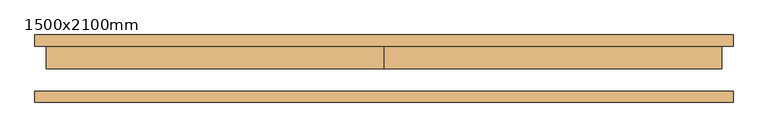
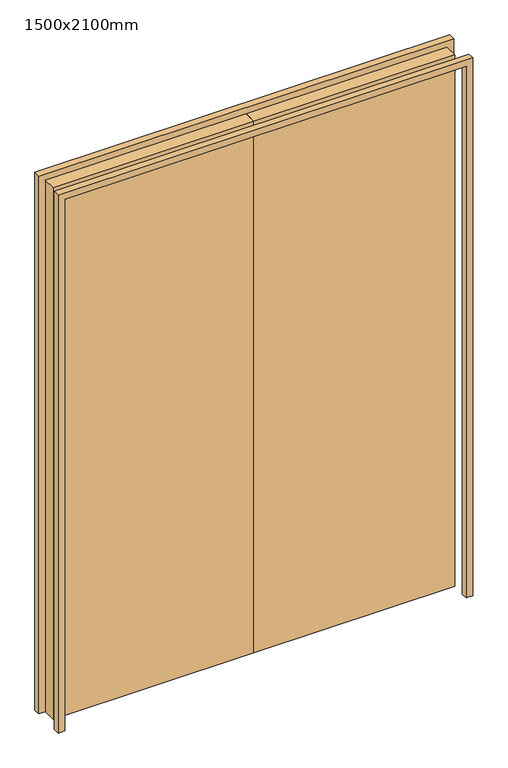
"""IFC4 building model written with IfcOpenShell, lengths in millimetres: door geometry, WWm-DoubleSolid-Flush : 1500x2100mm."""

from ifc_helpers import new_model, si_unit, frame, origin, origin_with_axes, place, context, project, spatial, polyline, outline, extrude, source, transform, mapped, element, save


def door_1500x2100mm_cd5236fe(model_context):
    return source(origin(), model_context, "Body", "SweptSolid", [
        extrude(outline(polyline([(0.0, 50.0), (750.0, 50.0), (750.0, 0.0), (0.0, 0.0), (0.0, 50.0)])), origin_with_axes(), (0.0, 0.0, 1.0), 2100.0),
        extrude(outline(polyline([(-750.0, 50.0), (0.0, 50.0), (0.0, 0.0), (-750.0, 0.0), (-750.0, 50.0)])), origin_with_axes(), (0.0, 0.0, 1.0), 2100.0),
        extrude(outline(polyline([(2100.0, -750.0), (2100.0, 750.0), (0.0, 750.0), (0.0, 775.0), (2125.0, 775.0), (2125.0, -775.0), (0.0, -775.0), (0.0, -750.0), (2100.0, -750.0)])), frame((0.0, -75.0, 0.0), z_axis=(0.0, 1.0, 0.0), x_axis=(0.0, 0.0, 1.0)), (0.0, 0.0, 1.0), 25.0),
        extrude(outline(polyline([(2100.0, -750.0), (2100.0, 750.0), (0.0, 750.0), (0.0, 775.0), (2125.0, 775.0), (2125.0, -775.0), (0.0, -775.0), (0.0, -750.0), (2100.0, -750.0)])), frame((0.0, 50.0, 0.0), z_axis=(0.0, 1.0, 0.0), x_axis=(0.0, 0.0, 1.0)), (0.0, 0.0, 1.0), 25.0),
    ])


if __name__ == "__main__":
    model = new_model("IFC4")
    model_context = context("Model", 3, world=origin())
    ifc_project = project(units=[si_unit("LENGTHUNIT", "METRE", prefix="MILLI")], contexts=[model_context])
    site = spatial("IfcSite", under=ifc_project)
    building = spatial("IfcBuilding", under=site)
    placement = place(None, origin())
    door_1500x2100mm_shape = door_1500x2100mm_cd5236fe(model_context)
    element("IfcDoor", 1, ObjectType="WWm-DoubleSolid-Flush : 1500x2100mm", at=placement, inside=building, context=model_context, shape_type="MappedRepresentation", body=[
        mapped(door_1500x2100mm_shape, transform((0.0, 0.0, 0.0), x_axis=(1.0, 0.0, 0.0), y_axis=(0.0, 1.0, 0.0), z_axis=(0.0, 0.0, 1.0))),
    ])
    save(model, "model.ifc")

# Revit data of these elements
# Type "WWm-DoubleSolid-Flush : 1500x2100mm"
#   Type Mark = "EX1-56"
#   Construction Type Id = "MDOOR"
#   Assembly Code = "C1020"
#   Analytic Construction = "Metal"
#   Thickness = 50 mm
#   Thermal Resistance (R) = 0.270117 (m²·K)/W
#   Heat Transfer Coefficient (U) = 3.7021 W/(m²·K)
#   Height = 2100 mm
#   Trim Projection Ext = 25 mm
#   Trim Projection Int = 25 mm
#   Trim Width = 25 mm
#   Width = 1500 mm
#   Not 90 Degree [instance default] = no
#   90 Degree [instance default] = yes
#   Door Material = WW-EC-RGB-White
#   Frame Material = WW-EC-RGB-White
#   Visual Light Transmittance = 0
#   Solar Heat Gain Coefficient = 0
#   Function = (empty or 0)
#   Wall Closure = (empty or 0)
# Element 1 (IfcDoor, "WWm-DoubleSolid-Flush : 1500x2100mm")
#   Materials on its faces: "WW-EC-RGB-White"
# Materials
#   "WW-EC-RGB-White": class "Generic", colour RGB 255 255 255, transparency 0, Comments = "If region requests off-white, swith asset color to RGB 231-228-220", Description = "Generic Color", Cost = 0
